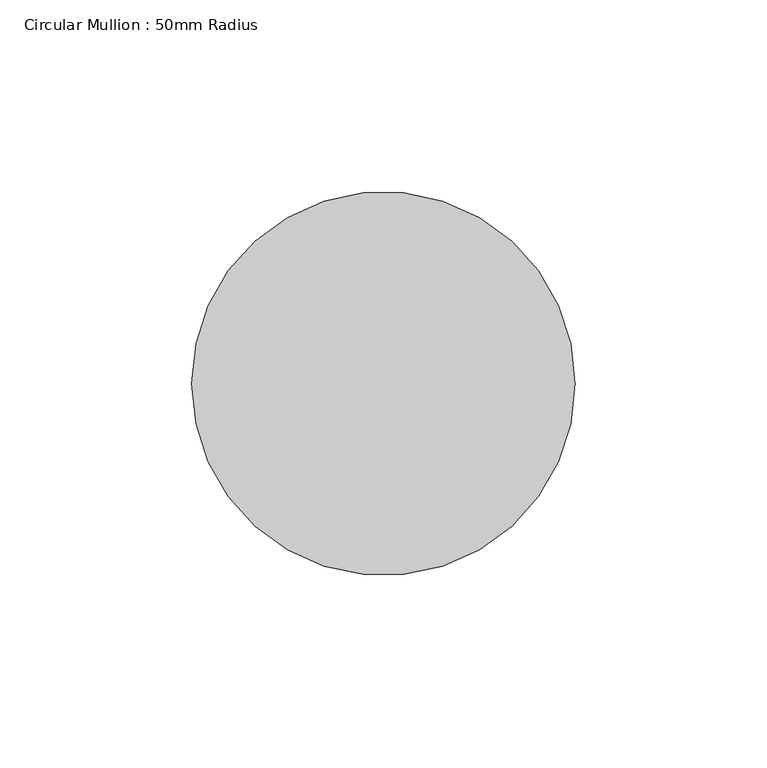
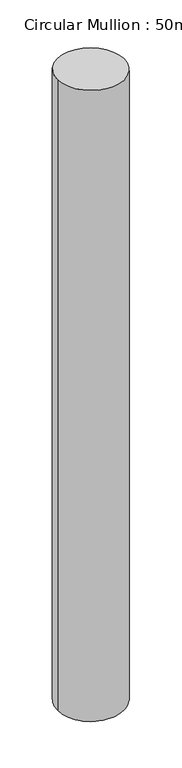
"""IFC4 building model written with IfcOpenShell, lengths in millimetres: member geometry, Circular Mullion : 50mm Radius."""

from ifc_helpers import new_model, si_unit, frame, origin, place, context, project, spatial, ellipse_curve, source, transform, mapped, element, save
from ifc_brep_helpers import plane_surface, cylinder_surface, advanced_brep


def circular_mullion_50mm_radius_3167f672(model_context):
    return source(origin(), model_context, "Body", "AdvancedBrep", [
        advanced_brep(
        [(-100.0, 0.0, 1.7229774), (0.0, 0.0, 0.0), (0.0, 0.0, -1000.0185569), (-100.0, 0.0, -1001.7393973)],
        [
            (0, 1, ellipse_curve(frame((-50.0, 0.0, 0.8614887), z_axis=(-0.01722543601620334, -0.014377392952704354, -0.9997482557753903), x_axis=(-0.7675266386424764, -0.6406242532874609, 0.022437136048629833)), 50.0125904, 50.0)),
            (1, 2),
            (2, 3, ellipse_curve(frame((-50.0, 0.0, -1000.8789771), z_axis=(-0.017204082439673522, -0.014359569963467942, 0.9997488796182135), x_axis=(0.7675271175790238, 0.6406246530369467, 0.022409321768563095)), 50.0125592, 50.0)),
            (3, 0),
            (1, 0, ellipse_curve(frame((-50.0, 0.0, 0.8614887), z_axis=(-0.01722543601620334, -0.014377392952704354, -0.9997482557753903), x_axis=(-0.7675266386424764, -0.6406242532874609, 0.022437136048629833)), 50.0125904, 50.0)),
            (3, 2, ellipse_curve(frame((-50.0, 0.0, -1000.8789771), z_axis=(-0.017204082439673522, -0.014359569963467942, 0.9997488796182135), x_axis=(0.7675271175790238, 0.6406246530369467, 0.022409321768563095)), 50.0125592, 50.0)),
        ],
        [
            cylinder_surface(frame((-50.0, 0.0, 0.0), z_axis=(0.0, 0.0, 1.0), x_axis=(1.0, 0.0, 0.0)), 50.0),
            plane_surface(frame((-195.3114409, 234.0010279, 0.0), z_axis=(0.01722543601620334, 0.014377392952704354, 0.9997482557753903), x_axis=(0.7675266386424765, 0.6406242532874606, -0.02243713604863125))),
            plane_surface(frame((-195.3114409, 234.0010279, -1000.0185569), z_axis=(0.017204082439673526, 0.014359569963467945, -0.9997488796182137), x_axis=(0.7675271175790239, 0.6406246530369468, 0.022409321768559035))),
        ],
        [
            (0, [[1, 2, 3, 4]]),
            (0, [[5, -4, 6, -2]]),
            (1, [[-1, -5]]),
            (2, [[-6, -3]]),
        ],
    ),
    ])


if __name__ == "__main__":
    model = new_model("IFC4")
    model_context = context("Model", 3, world=origin())
    ifc_project = project(units=[si_unit("LENGTHUNIT", "METRE", prefix="MILLI")], contexts=[model_context])
    site = spatial("IfcSite", under=ifc_project)
    building = spatial("IfcBuilding", under=site)
    placement = place(None, origin())
    circular_mullion_50mm_radius_shape = circular_mullion_50mm_radius_3167f672(model_context)
    element("IfcMember", 1, ObjectType="Circular Mullion : 50mm Radius", at=placement, inside=building, context=model_context, shape_type="MappedRepresentation", body=[
        mapped(circular_mullion_50mm_radius_shape, transform((0.0, 0.0, 0.0), x_axis=(1.0, 0.0, 0.0), y_axis=(0.0, 1.0, 0.0), z_axis=(0.0, 0.0, 1.0))),
    ])
    save(model, "model.ifc")

# Revit data of these elements
# Type "Circular Mullion : 50mm Radius"
#   built-in parameter 1007350 = 0.164042 (stored number, unit not read)
# Element 1 (IfcMember, "Circular Mullion : 50mm Radius")
#   Materials on its faces: "Aluminium"
# Materials
#   "Aluminium": class "Metal", colour RGB 247 247 247, transparency 0, Description = "Aluminium 6061", Cost = 0
